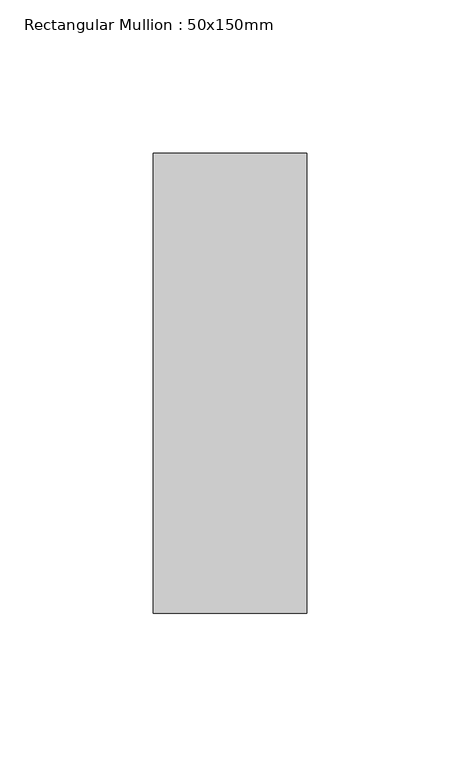
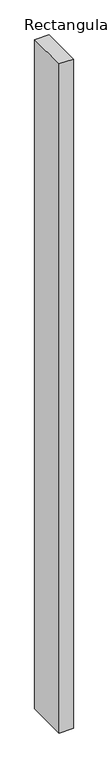
"""IFC4 building model written with IfcOpenShell, lengths in millimetres: member geometry, Rectangular Mullion : 50x150mm."""

import ifcopenshell
import ifcopenshell.guid

model = None  # the IFC model being written
_history = None  # IfcOwnerHistory: only IFC2X3 demands one
_inside = {}  # id of a spatial element -> (the spatial element, [elements in it])
_under = {}  # id of a project, library or spatial element -> (it, [spatial elements below it])
_declared = {}  # id of a project -> (the project, [libraries it declares])
_typed = {}  # id of a type object -> (the type object, [elements of that type])
_made_of = {}  # id of a material, layer set ... -> (it, [elements and type objects made of it])


def new_model(schema):
    """Start an empty IFC model of exactly this schema.

    Asked for "IFC4X3", IfcOpenShell would pick the latest addendum, in which some entities
    have other attributes; the version numbers below select the first issue.
    IFC2X3 requires an IfcOwnerHistory on every rooted entity: one is made here for all.
    """
    global model, _history
    if schema == "IFC4X3":
        model = ifcopenshell.file(schema_version=(4, 3, 0, 0))
    else:
        model = ifcopenshell.file(schema=schema)
    _inside.clear()
    _under.clear()
    _declared.clear()
    _typed.clear()
    _made_of.clear()
    _history = None
    if model.schema == "IFC2X3":
        org = make("IfcOrganization", Name="unknown")
        user = make(
            "IfcPersonAndOrganization",
            ThePerson=make("IfcPerson", FamilyName="unknown"),
            TheOrganization=org,
        )
        app = make(
            "IfcApplication",
            ApplicationDeveloper=org,
            Version="unknown",
            ApplicationFullName="unknown",
            ApplicationIdentifier="unknown",
        )
        _history = make(
            "IfcOwnerHistory",
            OwningUser=user,
            OwningApplication=app,
            ChangeAction="ADDED",
            CreationDate=0,
        )
    return model


def make(cls, **values):
    """One entity of the class cls with the attributes given. An attribute that is None is left unset."""
    return model.create_entity(
        cls, **{name: value for name, value in values.items() if value is not None}
    )


def rooted(cls, **values):
    """An entity with a GlobalId (a new one), such as an element, a storey or a relation."""
    return make(cls, GlobalId=ifcopenshell.guid.new(), OwnerHistory=_history, **values)


def si_unit(unit_type, name, prefix=None):
    """IfcSIUnit, for example si_unit("LENGTHUNIT", "METRE", prefix="MILLI")."""
    return make("IfcSIUnit", UnitType=unit_type, Prefix=prefix, Name=name)


def assignment(units):
    """IfcUnitAssignment: the units of a project."""
    return None if units is None else make("IfcUnitAssignment", Units=units)


def point(xyz):
    """IfcCartesianPoint."""
    return None if xyz is None else make("IfcCartesianPoint", Coordinates=xyz)


def direction(xyz):
    """IfcDirection."""
    return None if xyz is None else make("IfcDirection", DirectionRatios=xyz)


def frame(location, z_axis=None, x_axis=None):
    """IfcAxis2Placement3D, a coordinate frame: its origin and axes. An axis left out is left unset."""
    return make(
        "IfcAxis2Placement3D",
        Location=point(location),
        Axis=direction(z_axis),
        RefDirection=direction(x_axis),
    )


def origin():
    """The frame at (0, 0, 0) with its axes left unset."""
    return frame((0.0, 0.0, 0.0))


def place(relative_to, where):
    """IfcLocalPlacement: puts the frame where relative to a parent placement (None: the world)."""
    return make(
        "IfcLocalPlacement", PlacementRelTo=relative_to, RelativePlacement=where
    )


def context(
    kind, dimensions, precision=None, world=None, true_north=None, identifier=None
):
    """IfcGeometricRepresentationContext, for example the 3D "Model" context."""
    return make(
        "IfcGeometricRepresentationContext",
        ContextIdentifier=identifier,
        ContextType=kind,
        CoordinateSpaceDimension=dimensions,
        Precision=precision,
        WorldCoordinateSystem=world,
        TrueNorth=true_north,
    )


def project(units=None, contexts=None):
    """IfcProject with its units and contexts."""
    return rooted(
        "IfcProject",
        Name="project",
        RepresentationContexts=contexts,
        UnitsInContext=assignment(units),
    )


def spatial(cls, under=None, at=None, **own):
    """A site, building, storey or space (cls), placed at a placement, below another one or the project."""
    s = rooted(cls, ObjectPlacement=at, **own)
    if under is not None:
        _under.setdefault(under.id(), (under, []))[1].append(s)
    return s


def polyline(points):
    """IfcPolyline through the points."""
    return make("IfcPolyline", Points=[point(p) for p in points])


def outline(outer, holes=None, kind="AREA"):
    """IfcArbitraryClosedProfileDef: a profile drawn as a closed curve; with holes, ...WithVoids."""
    if holes is None:
        return make("IfcArbitraryClosedProfileDef", ProfileType=kind, OuterCurve=outer)
    return make(
        "IfcArbitraryProfileDefWithVoids",
        ProfileType=kind,
        OuterCurve=outer,
        InnerCurves=holes,
    )


def extrude(swept, where, along, depth):
    """IfcExtrudedAreaSolid: the profile swept, set in the frame where, extruded along a direction by depth."""
    return make(
        "IfcExtrudedAreaSolid",
        SweptArea=swept,
        Position=where,
        ExtrudedDirection=direction(along),
        Depth=depth,
    )


def shape(context_of_items, identifier, shape_type, items):
    """IfcShapeRepresentation: the items that make up one representation, for example the "Body"."""
    return make(
        "IfcShapeRepresentation",
        ContextOfItems=context_of_items,
        RepresentationIdentifier=identifier,
        RepresentationType=shape_type,
        Items=items,
    )


def source(mapping_origin, context_of_items, identifier, shape_type, items):
    """IfcRepresentationMap: a shape defined once, which mapped items show again and again."""
    return make(
        "IfcRepresentationMap",
        MappingOrigin=mapping_origin,
        MappedRepresentation=shape(context_of_items, identifier, shape_type, items),
    )


def transform(
    local_origin,
    x_axis=None,
    y_axis=None,
    z_axis=None,
    scale=None,
    scale2=None,
    scale3=None,
    uniform=True,
):
    """IfcCartesianTransformationOperator3D, or its non-uniform kind. x_axis, y_axis, z_axis: its Axis1, 2, 3."""
    if uniform:
        return make(
            "IfcCartesianTransformationOperator3D",
            Axis1=direction(x_axis),
            Axis2=direction(y_axis),
            LocalOrigin=point(local_origin),
            Scale=scale,
            Axis3=direction(z_axis),
        )
    return make(
        "IfcCartesianTransformationOperator3DnonUniform",
        Axis1=direction(x_axis),
        Axis2=direction(y_axis),
        LocalOrigin=point(local_origin),
        Scale=scale,
        Axis3=direction(z_axis),
        Scale2=scale2,
        Scale3=scale3,
    )


def mapped(mapping_source, mapping_target):
    """IfcMappedItem: shows the shape of a source again, moved by a transform."""
    return make(
        "IfcMappedItem", MappingSource=mapping_source, MappingTarget=mapping_target
    )


def made_of(thing, what):
    """Note that an element or type object is made of a material, layer set ...; save() writes the relation."""
    if what is not None:
        _made_of.setdefault(what.id(), (what, []))[1].append(thing)
    return thing


def element(
    cls,
    number,
    at=None,
    inside=None,
    cuts=None,
    type_object=None,
    material=None,
    context=None,
    identifier="Body",
    shape_type=None,
    held_by="IfcProductDefinitionShape",
    body=None,
    shapes=None,
    **own,
):
    """One element of the class cls, such as IfcWall. Its Tag is "e" and its number.

    at: its placement. inside: the storey or other place that contains it. cuts: it is an
    opening in that element (IfcRelVoidsElement). A single representation is given by context,
    identifier, shape_type and body (its items); several are given by shapes. held_by: the class
    of the entity that holds the representations. save() writes the other relations.
    """
    e = rooted(cls, Tag="e%d" % number, ObjectPlacement=at, **own)
    if body is not None:
        shapes = [shape(context, identifier, shape_type, body)]
    if shapes is not None:
        e.Representation = make(held_by, Representations=shapes)
    if inside is not None:
        _inside.setdefault(inside.id(), (inside, []))[1].append(e)
    if cuts is not None:
        rooted(
            "IfcRelVoidsElement", RelatingBuildingElement=cuts, RelatedOpeningElement=e
        )
    if type_object is not None:
        _typed.setdefault(type_object.id(), (type_object, []))[1].append(e)
    return made_of(e, material)


def aggregate(whole, parts):
    """IfcRelAggregates: a whole, such as a stair, and the parts it consists of."""
    return rooted("IfcRelAggregates", RelatingObject=whole, RelatedObjects=parts)


def save(model, path):
    """Write the relations noted so far, then the file.

    IfcRelAggregates (storeys below a building ...), IfcRelContainedInSpatialStructure (elements
    in a storey), IfcRelDefinesByType, IfcRelAssociatesMaterial and IfcRelDeclares: one each for
    every whole, place, type object, material and project.
    """
    for whole, parts in _under.values():
        aggregate(whole, parts)
    for where, things in _inside.values():
        rooted(
            "IfcRelContainedInSpatialStructure",
            RelatedElements=things,
            RelatingStructure=where,
        )
    for kind, things in _typed.values():
        rooted("IfcRelDefinesByType", RelatedObjects=things, RelatingType=kind)
    for what, things in _made_of.values():
        rooted("IfcRelAssociatesMaterial", RelatedObjects=things, RelatingMaterial=what)
    for by, libraries in _declared.values():
        rooted("IfcRelDeclares", RelatingContext=by, RelatedDefinitions=libraries)
    model.write(path)


def rectangular_mullion_50x150mm_4c3b9bdb(model_context):
    return source(origin(), model_context, "Body", "SweptSolid", [
        extrude(outline(polyline([(0.0, 75.0), (0.0, -75.0), (-50.0, -75.0), (-50.0, 75.0), (0.0, 75.0)])), frame((0.0, 0.0, -2500.0), z_axis=(0.0, 0.0, 1.0), x_axis=(1.0, 0.0, 0.0)), (0.0, 0.0, 1.0), 2500.0),
    ])


if __name__ == "__main__":
    model = new_model("IFC4")
    model_context = context("Model", 3, world=origin())
    ifc_project = project(units=[si_unit("LENGTHUNIT", "METRE", prefix="MILLI")], contexts=[model_context])
    site = spatial("IfcSite", under=ifc_project)
    building = spatial("IfcBuilding", under=site)
    placement = place(None, origin())
    rectangular_mullion_50x150mm_shape = rectangular_mullion_50x150mm_4c3b9bdb(model_context)
    element("IfcMember", 1, ObjectType="Rectangular Mullion : 50x150mm", at=placement, inside=building, context=model_context, shape_type="MappedRepresentation", body=[
        mapped(rectangular_mullion_50x150mm_shape, transform((0.0, 0.0, 0.0), x_axis=(1.0, 0.0, 0.0), y_axis=(0.0, 1.0, 0.0), z_axis=(0.0, 0.0, 1.0))),
    ])
    save(model, "model.ifc")

# Revit data of these elements
# Type "Rectangular Mullion : 50x150mm"
#   Keynote = "H11"
#   built-in parameter 1007304 = 0.492126 (stored number, unit not read)
#   built-in parameter 1007301 = 0.082021 (stored number, unit not read)
#   built-in parameter 1007300 = 0.082021 (stored number, unit not read)
# Element 1 (IfcMember, "Rectangular Mullion : 50x150mm")
#   Materials on its faces: "Aluminium"
# Materials
#   "Aluminium": class "Metal", colour RGB 247 247 247, transparency 0, Description = "Aluminium 6061", Cost = 0
